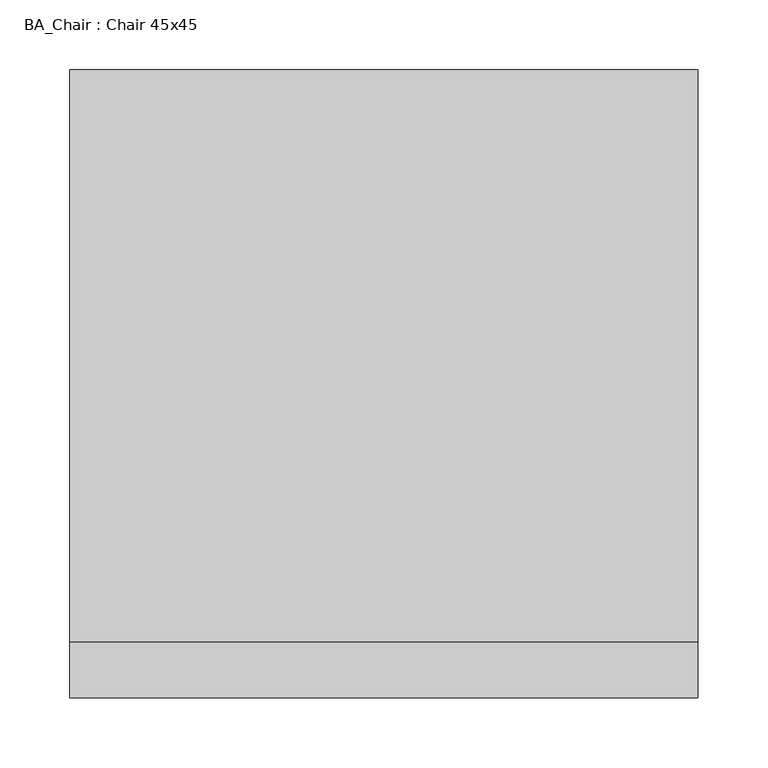
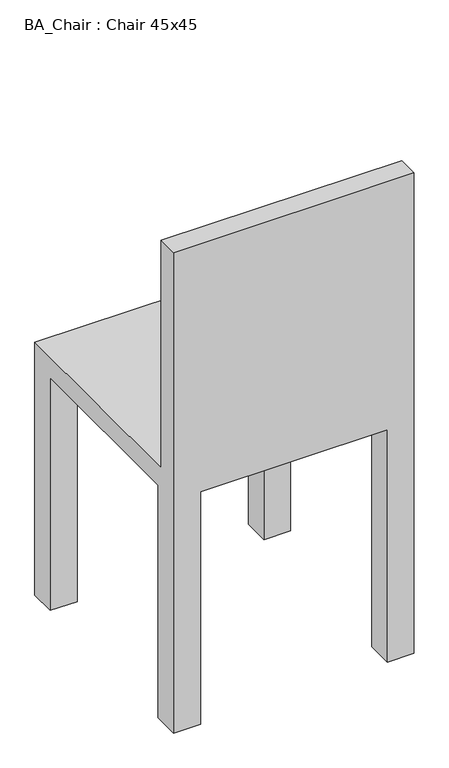
"""IFC4 building model written with IfcOpenShell, lengths in millimetres: furniture geometry, BA_Chair : Chair 45x45."""

from ifc_helpers import new_model, si_unit, origin, place, context, project, spatial, faceted_brep, source, transform, mapped, element, save


def ba_chair_chair_45x45_7c1e281b(model_context):
    return source(origin(), model_context, "Body", "Brep", [
        faceted_brep([(225.0, 225.0, 500.0), (225.0, -185.0, 500.0), (225.0, -185.0, 950.0), (225.0, -225.0, 950.0), (225.0, -225.0, 0.0), (225.0, -175.0, 0.0), (225.0, -175.0, 460.0), (225.0, 175.0, 460.0), (225.0, 175.0, 0.0), (225.0, 225.0, 0.0), (-225.0, -225.0, 950.0), (-225.0, -185.0, 950.0), (-225.0, -185.0, 500.0), (-225.0, 225.0, 500.0), (-225.0, 225.0, 0.0), (-225.0, 175.0, 0.0), (-225.0, 175.0, 460.0), (-225.0, -175.0, 460.0), (-225.0, -175.0, 0.0), (-225.0, -225.0, 0.0), (-175.0, -175.0, 460.0), (-175.0, 175.0, 460.0), (-175.0, 225.0, 460.0), (175.0, 225.0, 460.0), (175.0, 175.0, 460.0), (175.0, -175.0, 460.0), (175.0, -225.0, 460.0), (-175.0, -225.0, 460.0), (175.0, 225.0, 0.0), (-175.0, 225.0, 0.0), (-175.0, -225.0, 0.0), (175.0, -225.0, 0.0), (-175.0, -175.0, 0.0), (-175.0, 175.0, 0.0), (175.0, 175.0, 0.0), (175.0, -175.0, 0.0)], [[[0, 1, 2, 3, 4, 5, 6, 7, 8, 9]], [[10, 11, 12, 13, 14, 15, 16, 17, 18, 19]], [[20, 17, 16, 21, 22, 23, 24, 7, 6, 25, 26, 27]], [[13, 0, 9, 28, 23, 22, 29, 14]], [[1, 0, 13, 12]], [[2, 1, 12, 11]], [[3, 2, 11, 10]], [[4, 3, 10, 19, 30, 27, 26, 31]], [[32, 30, 19, 18]], [[32, 18, 17, 20]], [[30, 32, 20, 27]], [[29, 33, 15, 14]], [[15, 33, 21, 16]], [[33, 29, 22, 21]], [[9, 8, 34, 28]], [[28, 34, 24, 23]], [[34, 8, 7, 24]], [[5, 4, 31, 35]], [[5, 35, 25, 6]], [[35, 31, 26, 25]]]),
    ])


if __name__ == "__main__":
    model = new_model("IFC4")
    model_context = context("Model", 3, world=origin())
    ifc_project = project(units=[si_unit("LENGTHUNIT", "METRE", prefix="MILLI")], contexts=[model_context])
    site = spatial("IfcSite", under=ifc_project)
    building = spatial("IfcBuilding", under=site)
    placement = place(None, origin())
    ba_chair_chair_45x45_shape = ba_chair_chair_45x45_7c1e281b(model_context)
    element("IfcFurniture", 1, ObjectType="BA_Chair : Chair 45x45", at=placement, inside=building, context=model_context, shape_type="MappedRepresentation", body=[
        mapped(ba_chair_chair_45x45_shape, transform((0.0, 0.0, 0.0), x_axis=(1.0, 0.0, 0.0), y_axis=(0.0, 1.0, 0.0), z_axis=(0.0, 0.0, 1.0))),
    ])
    save(model, "model.ifc")

# Revit data of these elements
# Type "BA_Chair : Chair 45x45"
#   visina stolice = 500 mm
#   visina naslona = 450 mm
#   sirina/duzina stolice = 450 mm
#   Default Elevation = 0
# Element 1 (IfcFurniture, "BA_Chair : Chair 45x45")
#   Materials on its faces: "Default"
# Materials
#   "Default": class "Generic", colour RGB 255 255 255, transparency 0, Cost = 0
